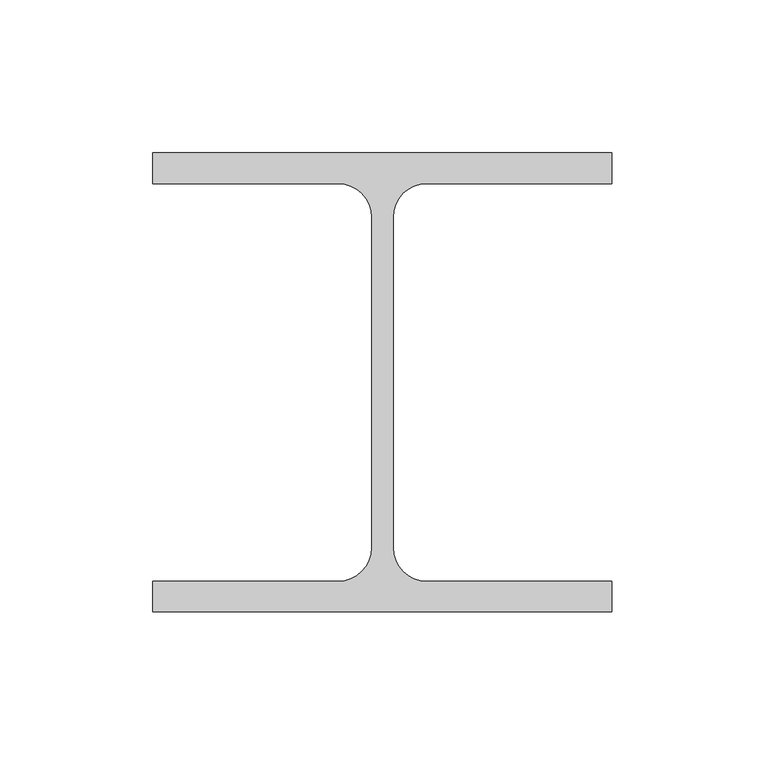
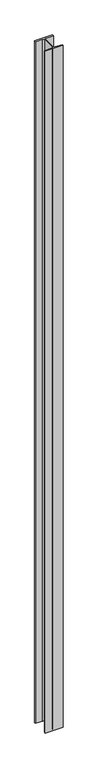
"""IFC4 building model written with IfcOpenShell, lengths in millimetres: column geometry, 0912_Steel Column_H_KSD3502 : H_SC_ASC_H-150x150x7x10."""

from ifc_helpers import new_model, si_unit, point, frame, frame_2d, origin, place, context, project, spatial, polyline, circle_curve, trimmed, segment, composite_curve, outline, extrude, source, transform, mapped, element, save


def column_5fc823e1(model_context):
    return source(origin(), model_context, "Body", "SweptSolid", [
        extrude(outline(composite_curve([segment(polyline([(75.0, 75.0), (75.0, 65.0), (14.5, 65.0)]), True, "CONTINUOUS"), segment(trimmed(circle_curve(frame_2d((14.5, 54.0)), 11.0), [point((14.5, 65.0))], [point((3.5, 54.0))], True, "CARTESIAN"), True, "CONTINUOUS"), segment(polyline([(3.5, 54.0), (3.5, -54.0)]), True, "CONTINUOUS"), segment(trimmed(circle_curve(frame_2d((14.5, -54.0)), 11.0), [point((3.5, -54.0))], [point((14.5, -65.0))], True, "CARTESIAN"), True, "CONTINUOUS"), segment(polyline([(14.5, -65.0), (75.0, -65.0), (75.0, -75.0), (-75.0, -75.0), (-75.0, -65.0), (-14.5, -65.0)]), True, "CONTINUOUS"), segment(trimmed(circle_curve(frame_2d((-14.5, -54.0)), 11.0), [point((-14.5, -65.0))], [point((-3.5, -54.0))], True, "CARTESIAN"), True, "CONTINUOUS"), segment(polyline([(-3.5, -54.0), (-3.5, 54.0)]), True, "CONTINUOUS"), segment(trimmed(circle_curve(frame_2d((-14.5, 54.0)), 11.0), [point((-3.5, 54.0))], [point((-14.5, 65.0))], True, "CARTESIAN"), True, "CONTINUOUS"), segment(polyline([(-14.5, 65.0), (-75.0, 65.0), (-75.0, 75.0), (75.0, 75.0)]), True, "CONTINUOUS")], self_intersect=False)), frame((0.0, 0.0, 599.9720055), z_axis=(0.0, 0.0, 1.0), x_axis=(1.0, 0.0, 0.0)), (0.0, 0.0, 1.0), 6000.0),
    ])


if __name__ == "__main__":
    model = new_model("IFC4")
    model_context = context("Model", 3, world=origin())
    ifc_project = project(units=[si_unit("LENGTHUNIT", "METRE", prefix="MILLI")], contexts=[model_context])
    site = spatial("IfcSite", under=ifc_project)
    building = spatial("IfcBuilding", under=site)
    placement = place(None, origin())
    column_shape = column_5fc823e1(model_context)
    element("IfcColumn", 1, ObjectType="0912_Steel Column_H_KSD3502 : H_SC_ASC_H-150x150x7x10", at=placement, inside=building, context=model_context, shape_type="MappedRepresentation", body=[
        mapped(column_shape, transform((0.0, 0.0, 0.0), x_axis=(1.0, 0.0, 0.0), y_axis=(0.0, 1.0, 0.0), z_axis=(0.0, 0.0, 1.0))),
    ])
    save(model, "model.ifc")

# Revit data of these elements
# Type "0912_Steel Column_H_KSD3502 : H_SC_ASC_H-150x150x7x10"
#   H_WM Code_1 = "S01AA002-00001 | Main Steel Structure Fabrication Work | Shelter/Building | Medium Steel - Standard (90KG/M>Weight≥30KG/M) | Material: (   )"
#   H_WM Code_2 = "S03AA028-00001 | Main Steel Structure Erection Work | Shelter/Building | Medium Steel (90KG/M>Weight≥30KG/M) | Material: (   )"
#   H_WM Code_3 = "S01AA010-00001 | Main Steel Structure Fabrication Work | Shelter/Building | Steel Painting/Coating | for Non-Fireproofed Steel Surface, Surface Preparation, Primer, Second & Final Coat | Material: (   )"
#   H_Q'ty Cal Type Tag = "SC-Q2"
#   Width = 15.0 cm
#   Web Thickness = 0.7 cm
#   Web Fillet = 1.1 cm
#   Warping Constant = 27562.5 cm⁶
#   Torsional Moment of Inertia = 11.6007 cm⁴
#   Section Area = 40.14 cm²
#   Plastic Modulus weak axis = 115.0 cm³
#   Plastic Modulus strong axis = 246.0 cm³
#   Perimeter = 0.87 m²/m
#   Nominal Weight = 31.50 kgf/m
#   Moment of Inertia weak axis = 563.00 cm⁴
#   Moment of Inertia strong axis = 1640.00 cm⁴
#   Height = 15.0 cm
#   Flange Thickness = 1.0 cm
#   Elastic Modulus weak axis = 75.1 cm³
#   Elastic Modulus strong axis = 219.0 cm³
#   Centroid Vertical = 7.5 cm
#   Centroid Horizontal = 7.5 cm
#   Structural Material [instance default] = Steel, 45-345
#   Section Name Key = ""
#   Bolt Spacing = 0
#   Assembly Code = ""
# Element 1 (IfcColumn, "0912_Steel Column_H_KSD3502 : H_SC_ASC_H-150x150x7x10")
#   Structural Material = A03AD029-00005_Anchor Bolt (Installation only)_M24
#   Materials on its faces: "A03AD029-00005_Anchor Bolt (Installation only)_M24"
# Materials
#   "Steel, 45-345": class "Metal", colour RGB 189 187 185, transparency 0, Description = "Steel 345 MPa", Cost = 0
#   "A03AD029-00005_Anchor Bolt (Installation only)_M24": class "Unassigned", colour RGB 84 83 81, transparency 0, Cost = 0
